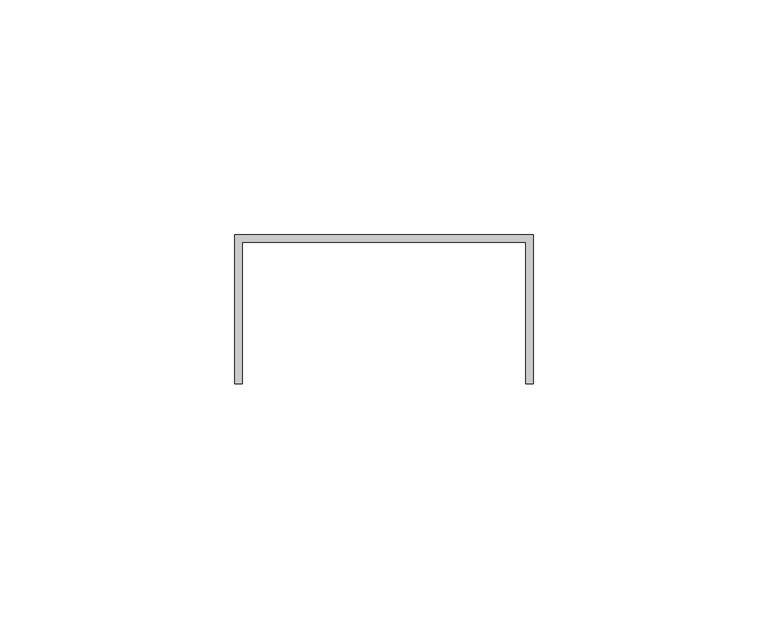
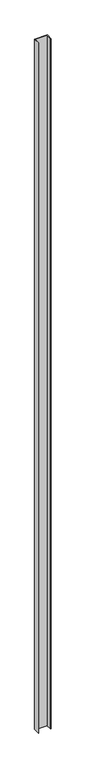
"""IFC4 building model written with IfcOpenShell, lengths in millimetres: proxy geometry, Generic Models 7:Generic Models 1:3:Generic Models 1:3 : Generic Models 7:Generic Models 1:305549:3:Generic Models 1:3:Generic Models 1:3 : Generic Models 7:Generic Models 1:305549:3 : Generic Models 7:Generic Models 1:3:Generic Models 1:3 : Generic Models 7:Generic Models 1:305549:301244:57 : Generic Models 7:Generic Models 1:3:Generic Models 1:3 : Generic Models 7:Generic Models 1:305549:3:Generic Models 1:3:Generic Models 1:3 : Generic Models 7:Generic Models 1:305549:3 : Generic Models 7:Generic Models 1:3:Generic Models 1:3 : Generic Models 7:Generic Models 1:305549:301244:308848."""

from ifc_helpers import new_model, si_unit, frame, origin, place, context, project, spatial, polyline, outline, extrude, source, transform, mapped, element, save


def generic_models_d71220d8(model_context):
    return source(origin(), model_context, "Body", "SweptSolid", [
        extrude(outline(polyline([(560352.9617239, -543227.3434586), (560352.9617239, -543259.0934586), (560351.3742239, -543259.0934586), (560351.3742239, -543228.9309586), (560291.0492239, -543228.9309586), (560291.0492239, -543259.0934586), (560289.4617239, -543259.0934586), (560289.4617239, -543227.3434586), (560352.9617239, -543227.3434586)])), frame((0.0, 0.0, 38.1), z_axis=(0.0, 0.0, 1.0), x_axis=(1.0, 0.0, 0.0)), (0.0, 0.0, 1.0), 3657.6),
    ])


if __name__ == "__main__":
    model = new_model("IFC4")
    model_context = context("Model", 3, world=origin())
    ifc_project = project(units=[si_unit("LENGTHUNIT", "METRE", prefix="MILLI")], contexts=[model_context])
    site = spatial("IfcSite", under=ifc_project)
    building = spatial("IfcBuilding", under=site)
    placement = place(None, origin())
    generic_models_shape = generic_models_d71220d8(model_context)
    element("IfcBuildingElementProxy", 1, Name="Generic Models 7:Generic Models 1:3:Generic Models 1:3 : Generic Models 7:Generic Models 1:305549:3:Generic Models 1:3:Generic Models 1:3 : Generic Models 7:Generic Models 1:305549:3 : Generic Models 7:Generic Models 1:3:Generic Models 1:3 : Generic Models 7:Generic Models 1:305549:301244:57 : Generic Models 7:Generic Models 1:3:Generic Models 1:3 : Generic Models 7:Generic Models 1:305549:3:Generic Models 1:3:Generic Models 1:3 : Generic Models 7:Generic Models 1:305549:3 : Generic Models 7:Generic Models 1:3:Generic Models 1:3 : Generic Models 7:Generic Models 1:305549:301244:308848", ObjectType="Generic Models 7:Generic Models 1:3:Generic Models 1:3 : Generic Models 7:Generic Models 1:305549:3:Generic Models 1:3:Generic Models 1:3 : Generic Models 7:Generic Models 1:305549:3 : Generic Models 7:Generic Models 1:3:Generic Models 1:3 : Generic Models 7:Generic Models 1:305549:301244:57 : Generic Models 7:Generic Models 1:3:Generic Models 1:3 : Generic Models 7:Generic Models 1:305549:3:Generic Models 1:3:Generic Models 1:3 : Generic Models 7:Generic Models 1:305549:3 : Generic Models 7:Generic Models 1:3:Generic Models 1:3 : Generic Models 7:Generic Models 1:305549:301244:308848", at=placement, inside=building, context=model_context, shape_type="MappedRepresentation", body=[
        mapped(generic_models_shape, transform((0.0, 0.0, 0.0), x_axis=(1.0, 0.0, 0.0), y_axis=(0.0, 1.0, 0.0), z_axis=(0.0, 0.0, 1.0))),
    ])
    save(model, "model.ifc")

# Revit data of these elements
# Type "Generic Models 7:Generic Models 1:3:Generic Models 1:3 : Generic Models 7:Generic Models 1:305549:3:Generic Models 1:3:Generic Models 1:3 : Generic Models 7:Generic Models 1:305549:3 : Generic Models 7:Generic Models 1:3:Generic Models 1:3 : Generic Models 7:Generic Models 1:305549:301244:57 : Generic Models 7:Generic Models 1:3:Generic Models 1:3 : Generic Models 7:Generic Models 1:305549:3:Generic Models 1:3:Generic Models 1:3 : Generic Models 7:Generic Models 1:305549:3 : Generic Models 7:Generic Models 1:3:Generic Models 1:3 : Generic Models 7:Generic Models 1:305549:301244:308848"
#   NameOverride = "Generic Models 7:Generic Models 1:3:Generic Models 1:3 : Generic Models 7:Generic Models 1:305549:3:Generic Models 1:3:Generic Models 1:3 : Generic Models 7:Generic Models 1:305549:3 : Generic Models 7:Generic Models 1:3:Generic Models 1:3 : Generic Models 7:Generic Models 1:305549:301244:308848"
#   ObjectTypeOverride = "Generic Models 1:3:Generic Models 1:3 : Generic Models 7:Generic Models 1:305549:3 : Generic Models 7:Generic Models 1:3:Generic Models 1:3 : Generic Models 7:Generic Models 1:305549:301244"
#   Reference = "Generic Models 1"
#   Tag = "308848"
# Element 1 (IfcBuildingElementProxy, "Generic Models 7:Generic Models 1:3:Generic Models 1:3 : Generic Models 7:Generic Models 1:305549:3:Generic Models 1:3:Generic Models 1:3 : Generic Models 7:Generic Models 1:305549:3 : Generic Models 7:Generic Models 1:3:Generic Models 1:3 : Generic Models 7:Generic Models 1:305549:301244:57 : Generic Models 7:Generic Models 1:3:Generic Models 1:3 : Generic Models 7:Generic Models 1:305549:3:Generic Models 1:3:Generic Models 1:3 : Generic Models 7:Generic Models 1:305549:3 : Generic Models 7:Generic Models 1:3:Generic Models 1:3 : Generic Models 7:Generic Models 1:305549:301244:308848")
#   Materials on its faces: "GALVANIZED U-CHANNEL (250T125-33)"
# Materials
#   "GALVANIZED U-CHANNEL (250T125-33)": class "Unassigned", colour RGB 202 201 200, transparency 0, Keynote = "M05451300.02", Cost = 0
